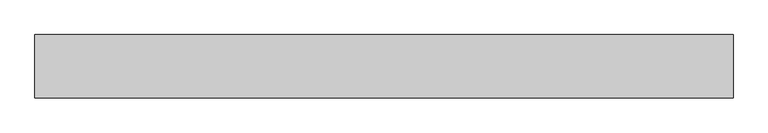
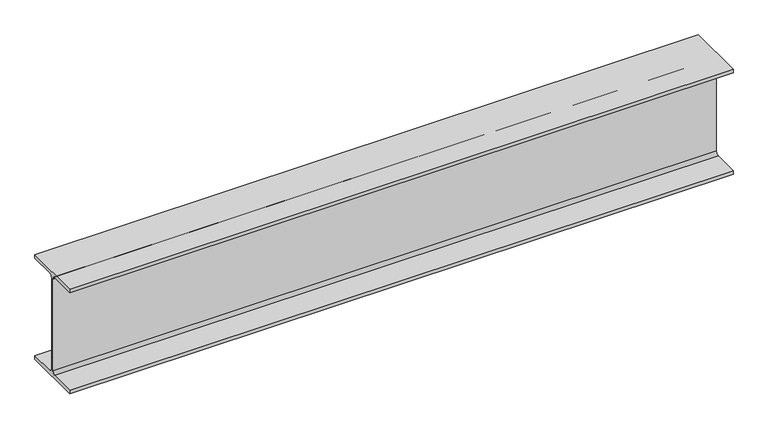
"""IFC4 building model written with IfcOpenShell, lengths in millimetres: beam geometry, Old_Steel Beam_H-KSD3502 : H_SB_ASB_H-200×200x8x12."""

from ifc_helpers import new_model, si_unit, point, frame, frame_2d, origin, place, context, project, spatial, polyline, circle_curve, trimmed, segment, composite_curve, outline, extrude, source, transform, mapped, element, save


def beam_3cc0a556(model_context):
    return source(origin(), model_context, "Body", "SweptSolid", [
        extrude(outline(composite_curve([segment(polyline([(82.5, -141.5), (82.5, -151.7), (-82.5, -151.7), (-82.5, -141.5), (-11.9, -141.5)]), True, "CONTINUOUS"), segment(trimmed(circle_curve(frame_2d((-11.9, -132.6)), 8.9), [point((-11.9, -141.5))], [point((-3.0, -132.6))], True, "CARTESIAN"), True, "CONTINUOUS"), segment(polyline([(-3.0, -132.6), (-3.0, 132.6)]), True, "CONTINUOUS"), segment(trimmed(circle_curve(frame_2d((-11.9, 132.6)), 8.9), [point((-3.0, 132.6))], [point((-11.9, 141.5))], True, "CARTESIAN"), True, "CONTINUOUS"), segment(polyline([(-11.9, 141.5), (-82.5, 141.5), (-82.5, 151.7), (82.5, 151.7), (82.5, 141.5), (11.9, 141.5)]), True, "CONTINUOUS"), segment(trimmed(circle_curve(frame_2d((11.9, 132.6)), 8.9), [point((11.9, 141.5))], [point((3.0, 132.6))], True, "CARTESIAN"), True, "CONTINUOUS"), segment(polyline([(3.0, 132.6), (3.0, -132.6)]), True, "CONTINUOUS"), segment(trimmed(circle_curve(frame_2d((11.9, -132.6)), 8.9), [point((3.0, -132.6))], [point((11.9, -141.5))], True, "CARTESIAN"), True, "CONTINUOUS"), segment(polyline([(11.9, -141.5), (82.5, -141.5)]), True, "CONTINUOUS")], self_intersect=False)), frame((-785.0333333, 0.0, 0.0), z_axis=(1.0, 0.0, 0.0), x_axis=(0.0, 1.0, 0.0)), (0.0, 0.0, 1.0), 1820.0666667),
    ])


if __name__ == "__main__":
    model = new_model("IFC4")
    model_context = context("Model", 3, world=origin())
    ifc_project = project(units=[si_unit("LENGTHUNIT", "METRE", prefix="MILLI")], contexts=[model_context])
    site = spatial("IfcSite", under=ifc_project)
    building = spatial("IfcBuilding", under=site)
    placement = place(None, origin())
    beam_shape = beam_3cc0a556(model_context)
    element("IfcBeam", 1, ObjectType="Old_Steel Beam_H-KSD3502 : H_SB_ASB_H-200×200x8x12", at=placement, inside=building, context=model_context, shape_type="MappedRepresentation", body=[
        mapped(beam_shape, transform((0.0, 0.0, 0.0), x_axis=(1.0, 0.0, 0.0), y_axis=(0.0, 1.0, 0.0), z_axis=(0.0, 0.0, 1.0))),
    ])
    save(model, "model.ifc")

# Revit data of these elements
# Type "Old_Steel Beam_H-KSD3502 : H_SB_ASB_H-200×200x8x12"
#   Width = 20.0 cm
#   Web Thickness = 0.8 cm
#   Web Fillet = 1.3 cm
#   Warping Constant = 141376.0 cm⁶
#   Torsional Moment of Inertia = 26.2485 cm⁴
#   Torsional Modulus = 1.0 cm³
#   Section Area = 63.53 cm²
#   Plastic Modulus weak axis = 244.0 cm³
#   Plastic Modulus strong axis = 525.0 cm³
#   Perimeter = 1.16 m²/m
#   Nominal Weight = 49.90 kgf/m
#   Moment of Inertia weak axis = 1600.00 cm⁴
#   Moment of Inertia strong axis = 4720.00 cm⁴
#   Height = 20.0 cm
#   Flange Thickness = 1.2 cm
#   Elastic Modulus weak axis = 160.0 cm³
#   Elastic Modulus strong axis = 472.0 cm³
#   Centroid Vertical = 10.0 cm
#   Centroid Horizontal = 10.0 cm
#   Length [instance default] = 1.5240 m
#   Structural Material [instance default] = Steel, 45-345
#   Assembly Code = ""
# Element 1 (IfcBeam, "Old_Steel Beam_H-KSD3502 : H_SB_ASB_H-200×200x8x12")
#   Structural Material = none
# Materials
#   "Steel, 45-345": class "Metal", colour RGB 189 187 185, transparency 0, Description = "Steel 345 MPa", Cost = 0
